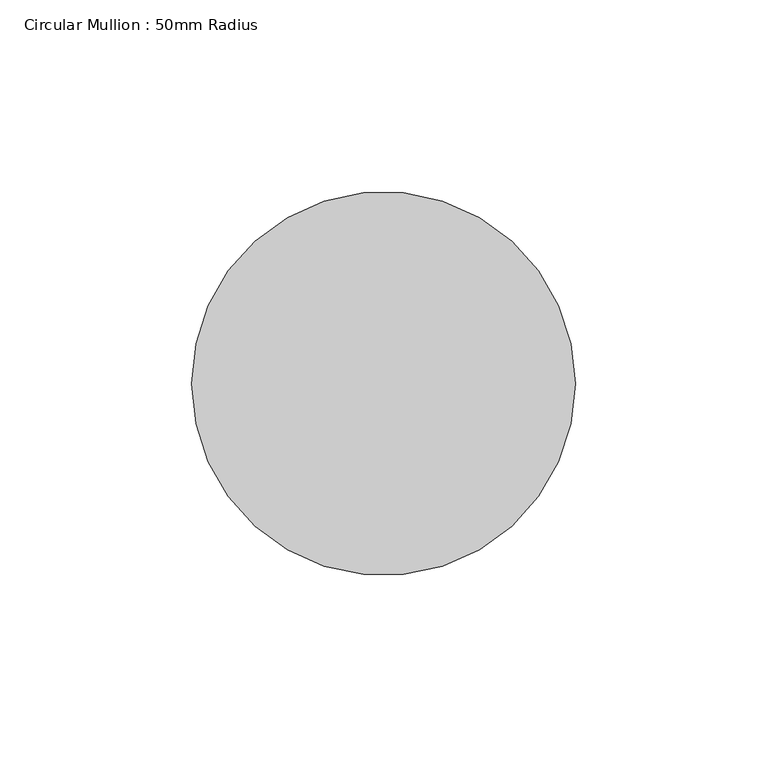
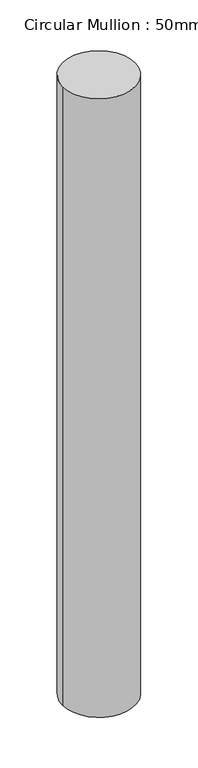
"""IFC4 building model written with IfcOpenShell, lengths in millimetres: member geometry, Circular Mullion : 50mm Radius."""

from ifc_helpers import new_model, si_unit, point, frame, origin, origin_2d, place, context, project, spatial, circle_curve, trimmed, segment, composite_curve, outline, extrude, source, transform, mapped, element, save


def circular_mullion_50mm_radius_48be029d(model_context):
    return source(origin(), model_context, "Body", "SweptSolid", [
        extrude(outline(composite_curve([segment(trimmed(circle_curve(origin_2d(), 50.0), [point((50.0, 0.0))], [point((-50.0, 0.0))], False, "CARTESIAN"), True, "CONTINUOUS"), segment(trimmed(circle_curve(origin_2d(), 50.0), [point((-50.0, 0.0))], [point((50.0, 0.0))], False, "CARTESIAN"), True, "CONTINUOUS")], self_intersect=False)), frame((0.0, 0.0, -901.7000767), z_axis=(0.0, 0.0, 1.0), x_axis=(1.0, 0.0, 0.0)), (0.0, 0.0, 1.0), 901.7000767),
    ])


if __name__ == "__main__":
    model = new_model("IFC4")
    model_context = context("Model", 3, world=origin())
    ifc_project = project(units=[si_unit("LENGTHUNIT", "METRE", prefix="MILLI")], contexts=[model_context])
    site = spatial("IfcSite", under=ifc_project)
    building = spatial("IfcBuilding", under=site)
    placement = place(None, origin())
    circular_mullion_50mm_radius_shape = circular_mullion_50mm_radius_48be029d(model_context)
    element("IfcMember", 1, ObjectType="Circular Mullion : 50mm Radius", at=placement, inside=building, context=model_context, shape_type="MappedRepresentation", body=[
        mapped(circular_mullion_50mm_radius_shape, transform((0.0, 0.0, 0.0), x_axis=(1.0, 0.0, 0.0), y_axis=(0.0, 1.0, 0.0), z_axis=(0.0, 0.0, 1.0))),
    ])
    save(model, "model.ifc")

# Revit data of these elements
# Type "Circular Mullion : 50mm Radius"
#   built-in parameter 1007350 = 0.164042 (stored number, unit not read)
# Element 1 (IfcMember, "Circular Mullion : 50mm Radius")
#   Materials on its faces: "Aluminium"
# Materials
#   "Aluminium": class "Metal", colour RGB 247 247 247, transparency 0, Description = "Aluminium 6061", Cost = 0
